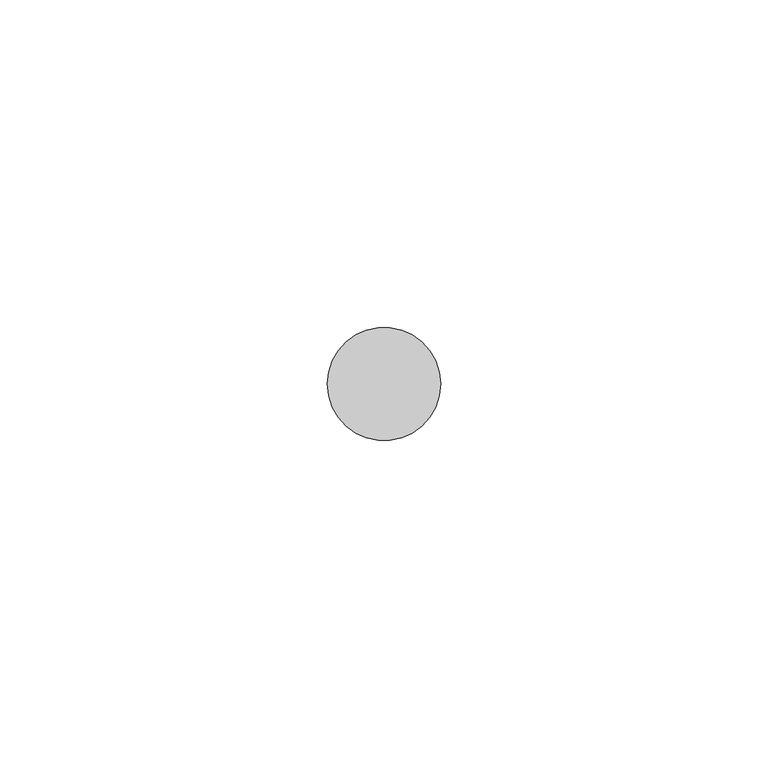
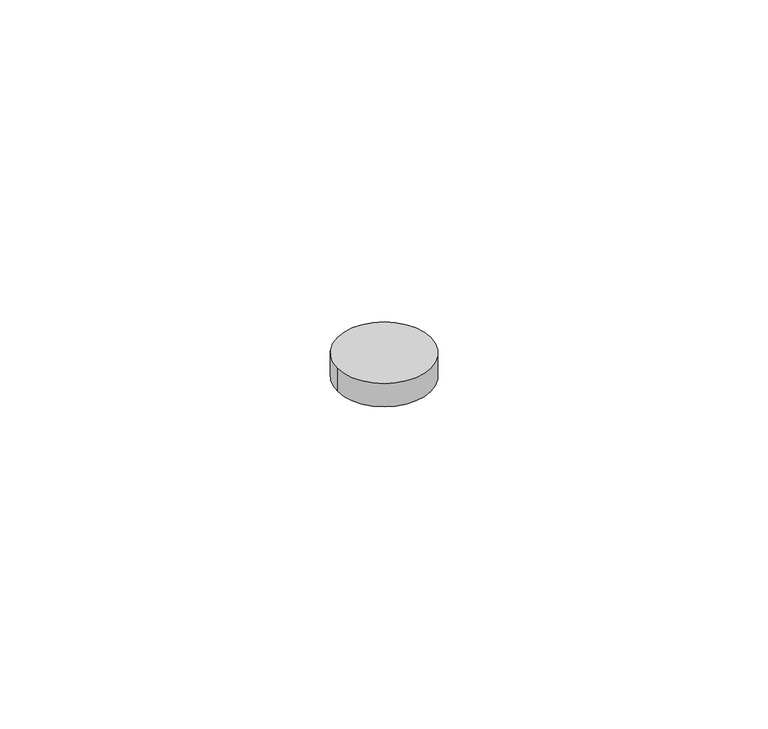
"""IFC4 building model written with IfcOpenShell, lengths in millimetres: proxy geometry, Hinge Pin Keeper : Hinge Pin Keeper."""

from ifc_helpers import new_model, si_unit, point, frame, frame_2d, origin, place, context, project, spatial, circle_curve, trimmed, segment, composite_curve, outline, extrude, source, transform, mapped, element, save


def generic_models_d25575f8(model_context):
    return source(origin(), model_context, "Body", "SweptSolid", [
        extrude(outline(composite_curve([segment(trimmed(circle_curve(frame_2d((587319.1320739, -531776.6049841)), 8.6534625), [point((587310.4786114, -531776.6049841))], [point((587327.7855364, -531776.6049841))], False, "CARTESIAN"), True, "CONTINUOUS"), segment(trimmed(circle_curve(frame_2d((587319.1320739, -531776.6049841)), 8.6534625), [point((587327.7855364, -531776.6049841))], [point((587310.4786114, -531776.6049841))], False, "CARTESIAN"), True, "CONTINUOUS")], self_intersect=False)), frame((0.0, 0.0, 458.9859375), z_axis=(0.0, 0.0, 1.0), x_axis=(1.0, 0.0, 0.0)), (0.0, 0.0, 1.0), 4.5640625),
    ])


if __name__ == "__main__":
    model = new_model("IFC4")
    model_context = context("Model", 3, world=origin())
    ifc_project = project(units=[si_unit("LENGTHUNIT", "METRE", prefix="MILLI")], contexts=[model_context])
    site = spatial("IfcSite", under=ifc_project)
    building = spatial("IfcBuilding", under=site)
    placement = place(None, origin())
    generic_models_shape = generic_models_d25575f8(model_context)
    element("IfcBuildingElementProxy", 1, Name="Hinge Pin Keeper : Hinge Pin Keeper", ObjectType="Hinge Pin Keeper : Hinge Pin Keeper", at=placement, inside=building, context=model_context, shape_type="MappedRepresentation", body=[
        mapped(generic_models_shape, transform((0.0, 0.0, 0.0), x_axis=(1.0, 0.0, 0.0), y_axis=(0.0, 1.0, 0.0), z_axis=(0.0, 0.0, 1.0))),
    ])
    save(model, "model.ifc")

# Revit data of these elements
# Element 1 (IfcBuildingElementProxy, "Hinge Pin Keeper : Hinge Pin Keeper")
#   Materials on its faces: "6\"X6\" WELD-ON STL BUTT HINGE"
# Materials
#   "6\"X6\" WELD-ON STL BUTT HINGE": class "Metal", colour RGB 189 187 185, transparency 0, Description = "Carbon steel", Cost = 0
